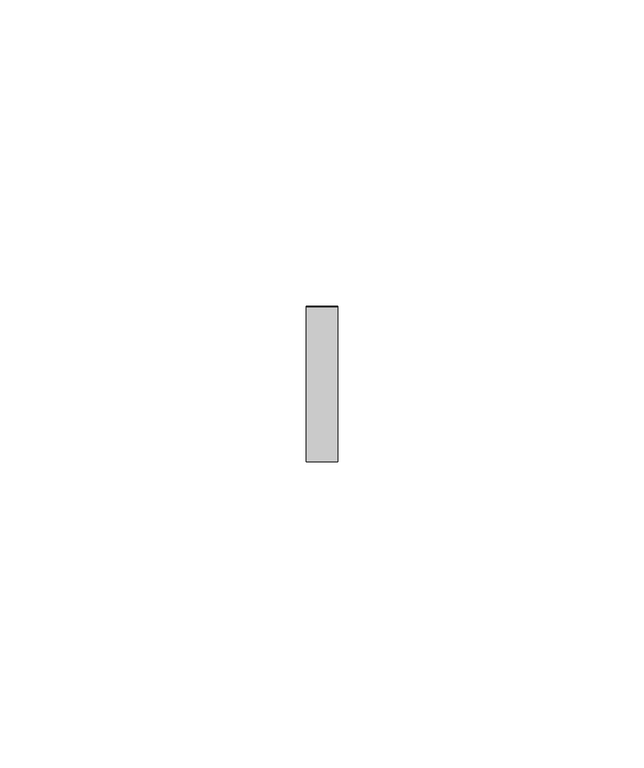
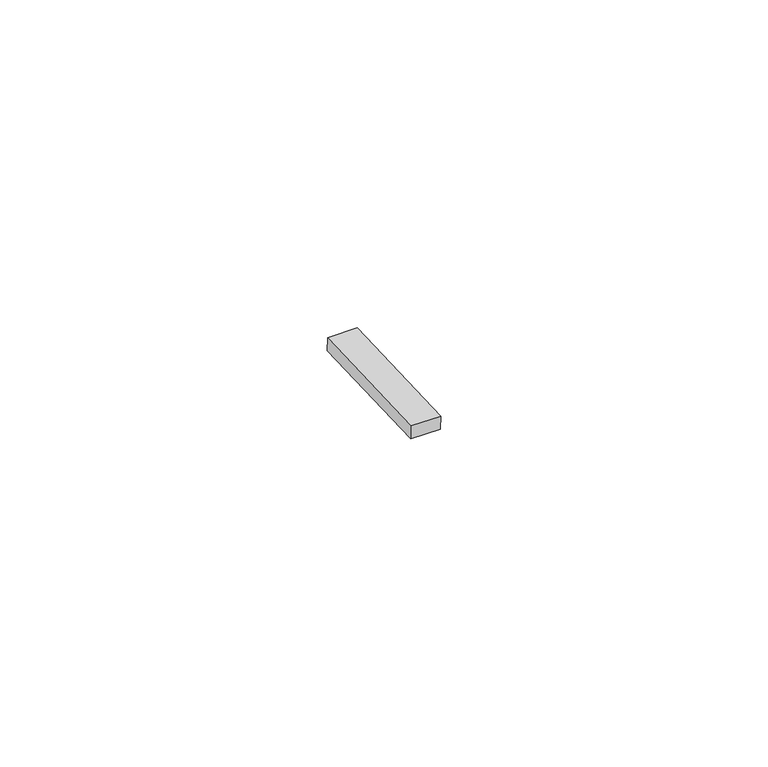
"""IFC4 building model written with IfcOpenShell, lengths in millimetres: proxy geometry, Inner panel:Inner panel:1:Inner panel:1 : Inner panel:Inner panel:300324:2:Inner panel:1:Inner panel:1 : Inner panel:Inner panel:300324:2 : Inner panel:Inner panel:1:Inner panel:1 : Inner panel:Inner panel:300324:300043:92 : Inner panel:Inner panel:1:Inner panel:1 : Inner panel:Inner panel:300324:2:Inner panel:1:Inner panel:1 : Inner panel:Inner panel:300324:2 : Inner panel:Inner panel:1:Inner panel:1 : Inner panel:Inner panel:300324:300043:308120."""

from ifc_helpers import new_model, si_unit, frame, origin, place, context, project, spatial, polyline, outline, extrude, source, transform, mapped, element, save


def generic_models_4b198137(model_context):
    return source(origin(), model_context, "Body", "SweptSolid", [
        extrude(outline(polyline([(0.0, -25.3999999), (0.0, 0.0), (5.2138089, 0.0), (5.2138089, -25.3999999), (0.0, -25.3999999)])), frame((592310.995117, -566905.6162814, 8857.0720004), z_axis=(0.0, -0.041630544712223896, 0.9991330730923502), x_axis=(-1.0, 0.0, 0.0)), (0.0, 0.0, 1.0), 2.4763745),
    ])


if __name__ == "__main__":
    model = new_model("IFC4")
    model_context = context("Model", 3, world=origin())
    ifc_project = project(units=[si_unit("LENGTHUNIT", "METRE", prefix="MILLI")], contexts=[model_context])
    site = spatial("IfcSite", under=ifc_project)
    building = spatial("IfcBuilding", under=site)
    placement = place(None, origin())
    generic_models_shape = generic_models_4b198137(model_context)
    element("IfcBuildingElementProxy", 1, Name="Inner panel:Inner panel:1:Inner panel:1 : Inner panel:Inner panel:300324:2:Inner panel:1:Inner panel:1 : Inner panel:Inner panel:300324:2 : Inner panel:Inner panel:1:Inner panel:1 : Inner panel:Inner panel:300324:300043:92 : Inner panel:Inner panel:1:Inner panel:1 : Inner panel:Inner panel:300324:2:Inner panel:1:Inner panel:1 : Inner panel:Inner panel:300324:2 : Inner panel:Inner panel:1:Inner panel:1 : Inner panel:Inner panel:300324:300043:308120", ObjectType="Inner panel:Inner panel:1:Inner panel:1 : Inner panel:Inner panel:300324:2:Inner panel:1:Inner panel:1 : Inner panel:Inner panel:300324:2 : Inner panel:Inner panel:1:Inner panel:1 : Inner panel:Inner panel:300324:300043:92 : Inner panel:Inner panel:1:Inner panel:1 : Inner panel:Inner panel:300324:2:Inner panel:1:Inner panel:1 : Inner panel:Inner panel:300324:2 : Inner panel:Inner panel:1:Inner panel:1 : Inner panel:Inner panel:300324:300043:308120", at=placement, inside=building, context=model_context, shape_type="MappedRepresentation", body=[
        mapped(generic_models_shape, transform((0.0, 0.0, 0.0), x_axis=(1.0, 0.0, 0.0), y_axis=(0.0, 1.0, 0.0), z_axis=(0.0, 0.0, 1.0))),
    ])
    save(model, "model.ifc")

# Revit data of these elements
# Type "Inner panel:Inner panel:1:Inner panel:1 : Inner panel:Inner panel:300324:2:Inner panel:1:Inner panel:1 : Inner panel:Inner panel:300324:2 : Inner panel:Inner panel:1:Inner panel:1 : Inner panel:Inner panel:300324:300043:92 : Inner panel:Inner panel:1:Inner panel:1 : Inner panel:Inner panel:300324:2:Inner panel:1:Inner panel:1 : Inner panel:Inner panel:300324:2 : Inner panel:Inner panel:1:Inner panel:1 : Inner panel:Inner panel:300324:300043:308120"
#   NameOverride = "Inner panel:Inner panel:1:Inner panel:1 : Inner panel:Inner panel:300324:2:Inner panel:1:Inner panel:1 : Inner panel:Inner panel:300324:2 : Inner panel:Inner panel:1:Inner panel:1 : Inner panel:Inner panel:300324:300043:308120"
#   ObjectTypeOverride = "Inner panel:1:Inner panel:1 : Inner panel:Inner panel:300324:2 : Inner panel:Inner panel:1:Inner panel:1 : Inner panel:Inner panel:300324:300043"
#   Reference = "Inner panel"
#   Tag = "308120"
# Element 1 (IfcBuildingElementProxy, "Inner panel:Inner panel:1:Inner panel:1 : Inner panel:Inner panel:300324:2:Inner panel:1:Inner panel:1 : Inner panel:Inner panel:300324:2 : Inner panel:Inner panel:1:Inner panel:1 : Inner panel:Inner panel:300324:300043:92 : Inner panel:Inner panel:1:Inner panel:1 : Inner panel:Inner panel:300324:2:Inner panel:1:Inner panel:1 : Inner panel:Inner panel:300324:2 : Inner panel:Inner panel:1:Inner panel:1 : Inner panel:Inner panel:300324:300043:308120")
#   Materials on its faces: "AT CLIP - 1\" WIDE NON ABSORBENT, WEATHER-RESISTANT NEOPRENE/EPDM/SBR FOAM"
# Materials
#   "AT CLIP - 1\" WIDE NON ABSORBENT, WEATHER-RESISTANT NEOPRENE/EPDM/SBR FOAM": class "Generic", colour RGB 85 85 85, transparency 0, Cost = 0
